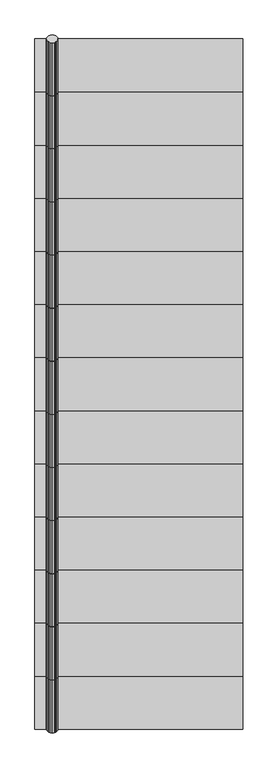
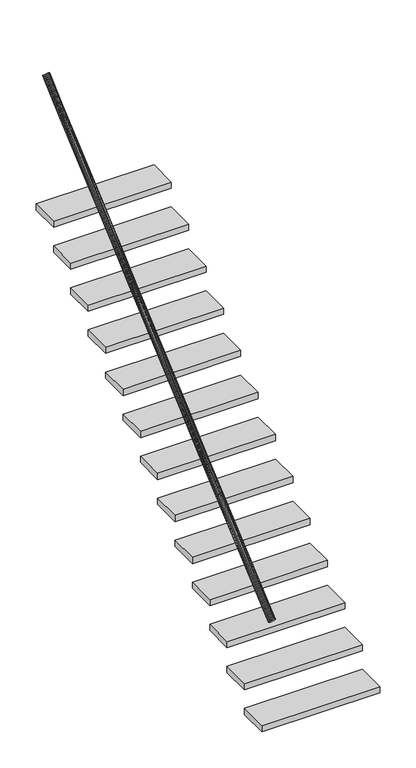
"""IFC4 building model written with IfcOpenShell, lengths in millimetres: stair geometry, 0_3d."""

from ifc_helpers import new_model, si_unit, frame, origin, origin_with_axes, place, context, project, spatial, polyline, outline, extrude, source, transform, mapped, element, save


def stair_2233e0a3(model_context):
    return source(origin(), model_context, "Body", "SweptSolid", [
        extrude(outline(polyline([(1.2235871, -7.9923214), (0.0, 0.0), (1.2235871, 7.9923214), (4.7745751, 15.2022986), (10.3053687, 20.924169), (17.2745751, 24.5978359), (25.0, 25.8636953), (32.7254249, 24.5978359), (39.6946313, 20.924169), (45.2254249, 15.2022986), (48.7764129, 7.9923214), (50.0, 0.0), (48.7764129, -7.9923214), (45.2254249, -15.2022986), (39.6946313, -20.9241691), (32.7254249, -24.5978359), (25.0, -25.8636953), (17.2745751, -24.5978359), (10.3053687, -20.9241691), (4.7745751, -15.2022986), (1.2235871, -7.9923214)])), frame((100.0, 246.9712063, 1069.5592366), z_axis=(0.0, 0.7546055221634433, 0.6561787149248571), x_axis=(-1.0, 0.0, 0.0)), (0.0, 0.0, 1.0), 304.7950131),
        extrude(outline(polyline([(1.2235871, -7.9923214), (0.0, 0.0), (1.2235871, 7.9923214), (4.7745751, 15.2022986), (10.3053687, 20.924169), (17.2745751, 24.5978359), (25.0, 25.8636953), (32.7254249, 24.5978359), (39.6946313, 20.924169), (45.2254249, 15.2022986), (48.7764129, 7.9923214), (50.0, 0.0), (48.7764129, -7.9923214), (45.2254249, -15.2022986), (39.6946313, -20.9241691), (32.7254249, -24.5978359), (25.0, -25.8636953), (17.2745751, -24.5978359), (10.3053687, -20.9241691), (4.7745751, -15.2022986), (1.2235871, -7.9923214)])), frame((100.0, 1396.9712063, 2069.5592366), z_axis=(0.0, 0.7546055221634361, 0.6561787149248655), x_axis=(-1.0, 0.0, 0.0)), (0.0, 0.0, 1.0), 304.7950131),
        extrude(outline(polyline([(0.0, 1856.9712063), (0.0, 2086.9712063), (900.0, 2086.9712063), (900.0, 1856.9712063), (0.0, 1856.9712063)])), frame((0.0, 0.0, 1600.0), z_axis=(0.0, 0.0, 1.0), x_axis=(1.0, 0.0, 0.0)), (0.0, 0.0, 1.0), 50.0),
        extrude(outline(polyline([(0.0, 2086.9712063), (0.0, 2316.9712063), (900.0, 2316.9712063), (900.0, 2086.9712063), (0.0, 2086.9712063)])), frame((0.0, 0.0, 1800.0), z_axis=(0.0, 0.0, 1.0), x_axis=(1.0, 0.0, 0.0)), (0.0, 0.0, 1.0), 50.0),
        extrude(outline(polyline([(1.2235871, -7.9923214), (0.0, 0.0), (1.2235871, 7.9923214), (4.7745751, 15.2022986), (10.3053687, 20.924169), (17.2745751, 24.5978359), (25.0, 25.8636953), (32.7254249, 24.5978359), (39.6946313, 20.924169), (45.2254249, 15.2022986), (48.7764129, 7.9923214), (50.0, 0.0), (48.7764129, -7.9923214), (45.2254249, -15.2022986), (39.6946313, -20.9241691), (32.7254249, -24.5978359), (25.0, -25.8636953), (17.2745751, -24.5978359), (10.3053687, -20.9241691), (4.7745751, -15.2022986), (1.2235871, -7.9923214)])), frame((100.0, 1166.9712063, 1869.5592366), z_axis=(0.0, 0.7546055221634385, 0.656178714924863), x_axis=(-1.0, 0.0, 0.0)), (0.0, 0.0, 1.0), 304.7950131),
        extrude(outline(polyline([(0.0, 936.9712063), (0.0, 1166.9712063), (900.0, 1166.9712063), (900.0, 936.9712063), (0.0, 936.9712063)])), frame((0.0, 0.0, 800.0), z_axis=(0.0, 0.0, 1.0), x_axis=(1.0, 0.0, 0.0)), (0.0, 0.0, 1.0), 50.0),
        extrude(outline(polyline([(0.0, 2546.9712063), (0.0, 2776.9712063), (900.0, 2776.9712063), (900.0, 2546.9712063), (0.0, 2546.9712063)])), frame((0.0, 0.0, 2200.0), z_axis=(0.0, 0.0, 1.0), x_axis=(1.0, 0.0, 0.0)), (0.0, 0.0, 1.0), 50.0),
        extrude(outline(polyline([(0.0, 1626.9712063), (0.0, 1856.9712063), (900.0, 1856.9712063), (900.0, 1626.9712063), (0.0, 1626.9712063)])), frame((0.0, 0.0, 1400.0), z_axis=(0.0, 0.0, 1.0), x_axis=(1.0, 0.0, 0.0)), (0.0, 0.0, 1.0), 50.0),
        extrude(outline(polyline([(0.0, 1166.9712063), (0.0, 1396.9712063), (900.0, 1396.9712063), (900.0, 1166.9712063), (0.0, 1166.9712063)])), frame((0.0, 0.0, 1000.0), z_axis=(0.0, 0.0, 1.0), x_axis=(1.0, 0.0, 0.0)), (0.0, 0.0, 1.0), 50.0),
        extrude(outline(polyline([(0.0, 246.9712063), (0.0, 476.9712063), (900.0, 476.9712063), (900.0, 246.9712063), (0.0, 246.9712063)])), frame((0.0, 0.0, 200.0), z_axis=(0.0, 0.0, 1.0), x_axis=(1.0, 0.0, 0.0)), (0.0, 0.0, 1.0), 50.0),
        extrude(outline(polyline([(0.0, 1396.9712063), (0.0, 1626.9712063), (900.0, 1626.9712063), (900.0, 1396.9712063), (0.0, 1396.9712063)])), frame((0.0, 0.0, 1200.0), z_axis=(0.0, 0.0, 1.0), x_axis=(1.0, 0.0, 0.0)), (0.0, 0.0, 1.0), 50.0),
        extrude(outline(polyline([(1.2235871, -7.9923214), (0.0, 0.0), (1.2235871, 7.9923214), (4.7745751, 15.2022986), (10.3053687, 20.924169), (17.2745751, 24.5978359), (25.0, 25.8636953), (32.7254249, 24.5978359), (39.6946313, 20.924169), (45.2254249, 15.2022986), (48.7764129, 7.9923214), (50.0, 0.0), (48.7764129, -7.9923214), (45.2254249, -15.2022986), (39.6946313, -20.9241691), (32.7254249, -24.5978359), (25.0, -25.8636953), (17.2745751, -24.5978359), (10.3053687, -20.9241691), (4.7745751, -15.2022986), (1.2235871, -7.9923214)])), frame((100.0, 1856.9712063, 2469.5592366), z_axis=(0.0, 0.7546055221634393, 0.6561787149248619), x_axis=(-1.0, 0.0, 0.0)), (0.0, 0.0, 1.0), 304.7950131),
        extrude(outline(polyline([(1.2235871, -7.9923214), (0.0, 0.0), (1.2235871, 7.9923214), (4.7745751, 15.2022986), (10.3053687, 20.924169), (17.2745751, 24.5978359), (25.0, 25.8636953), (32.7254249, 24.5978359), (39.6946313, 20.924169), (45.2254249, 15.2022986), (48.7764129, 7.9923214), (50.0, 0.0), (48.7764129, -7.9923214), (45.2254249, -15.2022986), (39.6946313, -20.9241691), (32.7254249, -24.5978359), (25.0, -25.8636953), (17.2745751, -24.5978359), (10.3053687, -20.9241691), (4.7745751, -15.2022986), (1.2235871, -7.9923214)])), frame((100.0, 1626.9712063, 2269.5592366), z_axis=(0.0, 0.7546055221634641, 0.6561787149248334), x_axis=(-1.0, 0.0, 0.0)), (0.0, 0.0, 1.0), 304.7950131),
        extrude(outline(polyline([(0.0, 2776.9712063), (0.0, 3006.9712063), (900.0, 3006.9712063), (900.0, 2776.9712063), (0.0, 2776.9712063)])), frame((0.0, 0.0, 2400.0), z_axis=(0.0, 0.0, 1.0), x_axis=(1.0, 0.0, 0.0)), (0.0, 0.0, 1.0), 50.0),
        extrude(outline(polyline([(0.0, 476.9712063), (0.0, 706.9712063), (900.0, 706.9712063), (900.0, 476.9712063), (0.0, 476.9712063)])), frame((0.0, 0.0, 400.0), z_axis=(0.0, 0.0, 1.0), x_axis=(1.0, 0.0, 0.0)), (0.0, 0.0, 1.0), 50.0),
        extrude(outline(polyline([(1.2235871, -7.9923214), (0.0, 0.0), (1.2235871, 7.9923214), (4.7745751, 15.2022986), (10.3053687, 20.924169), (17.2745751, 24.5978359), (25.0, 25.8636953), (32.7254249, 24.5978359), (39.6946313, 20.924169), (45.2254249, 15.2022986), (48.7764129, 7.9923214), (50.0, 0.0), (48.7764129, -7.9923214), (45.2254249, -15.2022986), (39.6946313, -20.9241691), (32.7254249, -24.5978359), (25.0, -25.8636953), (17.2745751, -24.5978359), (10.3053687, -20.9241691), (4.7745751, -15.2022986), (1.2235871, -7.9923214)])), frame((100.0, 706.9712063, 1469.5592366), z_axis=(0.0, 0.7546055221634701, 0.6561787149248264), x_axis=(-1.0, 0.0, 0.0)), (0.0, 0.0, 1.0), 304.7950131),
        extrude(outline(polyline([(1.2235871, -7.9923214), (0.0, 0.0), (1.2235871, 7.9923214), (4.7745751, 15.2022986), (10.3053687, 20.924169), (17.2745751, 24.5978359), (25.0, 25.8636953), (32.7254249, 24.5978359), (39.6946313, 20.924169), (45.2254249, 15.2022986), (48.7764129, 7.9923214), (50.0, 0.0), (48.7764129, -7.9923214), (45.2254249, -15.2022986), (39.6946313, -20.9241691), (32.7254249, -24.5978359), (25.0, -25.8636953), (17.2745751, -24.5978359), (10.3053687, -20.9241691), (4.7745751, -15.2022986), (1.2235871, -7.9923214)])), frame((100.0, 2086.9712063, 2669.5592366), z_axis=(0.0, 0.7546055221634421, 0.6561787149248586), x_axis=(-1.0, 0.0, 0.0)), (0.0, 0.0, 1.0), 304.7950131),
        extrude(outline(polyline([(1.2235871, -7.9923214), (0.0, 0.0), (1.2235871, 7.9923214), (4.7745751, 15.2022986), (10.3053687, 20.924169), (17.2745751, 24.5978359), (25.0, 25.8636953), (32.7254249, 24.5978359), (39.6946313, 20.924169), (45.2254249, 15.2022986), (48.7764129, 7.9923214), (50.0, 0.0), (48.7764129, -7.9923214), (45.2254249, -15.2022986), (39.6946313, -20.9241691), (32.7254249, -24.5978359), (25.0, -25.8636953), (17.2745751, -24.5978359), (10.3053687, -20.9241691), (4.7745751, -15.2022986), (1.2235871, -7.9923214)])), frame((100.0, 936.9712063, 1669.5592366), z_axis=(0.0, 0.7546055221634438, 0.6561787149248568), x_axis=(-1.0, 0.0, 0.0)), (0.0, 0.0, 1.0), 304.7950131),
        extrude(outline(polyline([(0.0, 706.9712063), (0.0, 936.9712063), (900.0, 936.9712063), (900.0, 706.9712063), (0.0, 706.9712063)])), frame((0.0, 0.0, 600.0), z_axis=(0.0, 0.0, 1.0), x_axis=(1.0, 0.0, 0.0)), (0.0, 0.0, 1.0), 50.0),
        extrude(outline(polyline([(1.2235871, -7.9923214), (0.0, 0.0), (1.2235871, 7.9923214), (4.7745751, 15.2022986), (10.3053687, 20.924169), (17.2745751, 24.5978359), (25.0, 25.8636953), (32.7254249, 24.5978359), (39.6946313, 20.924169), (45.2254249, 15.2022986), (48.7764129, 7.9923214), (50.0, 0.0), (48.7764129, -7.9923214), (45.2254249, -15.2022986), (39.6946313, -20.9241691), (32.7254249, -24.5978359), (25.0, -25.8636953), (17.2745751, -24.5978359), (10.3053687, -20.9241691), (4.7745751, -15.2022986), (1.2235871, -7.9923214)])), frame((100.0, 2316.9712063, 2869.5592366), z_axis=(0.0, 0.7546055221634657, 0.6561787149248317), x_axis=(-1.0, 0.0, 0.0)), (0.0, 0.0, 1.0), 304.7950131),
        extrude(outline(polyline([(1.2235871, -7.9923214), (0.0, 0.0), (1.2235871, 7.9923214), (4.7745751, 15.2022986), (10.3053687, 20.924169), (17.2745751, 24.5978359), (25.0, 25.8636953), (32.7254249, 24.5978359), (39.6946313, 20.924169), (45.2254249, 15.2022986), (48.7764129, 7.9923214), (50.0, 0.0), (48.7764129, -7.9923214), (45.2254249, -15.2022986), (39.6946313, -20.9241691), (32.7254249, -24.5978359), (25.0, -25.8636953), (17.2745751, -24.5978359), (10.3053687, -20.9241691), (4.7745751, -15.2022986), (1.2235871, -7.9923214)])), frame((100.0, 2776.9712063, 3269.5592366), z_axis=(0.0, 0.754605522163467, 0.65617871492483), x_axis=(-1.0, 0.0, 0.0)), (0.0, 0.0, 1.0), 304.7950131),
        extrude(outline(polyline([(1.2235871, -7.9923214), (0.0, 0.0), (1.2235871, 7.9923214), (4.7745751, 15.2022986), (10.3053687, 20.924169), (17.2745751, 24.5978359), (25.0, 25.8636953), (32.7254249, 24.5978359), (39.6946313, 20.924169), (45.2254249, 15.2022986), (48.7764129, 7.9923214), (50.0, 0.0), (48.7764129, -7.9923214), (45.2254249, -15.2022986), (39.6946313, -20.9241691), (32.7254249, -24.5978359), (25.0, -25.8636953), (17.2745751, -24.5978359), (10.3053687, -20.9241691), (4.7745751, -15.2022986), (1.2235871, -7.9923214)])), frame((100.0, 476.9712063, 1269.5592366), z_axis=(0.0, 0.7546055221634442, 0.6561787149248562), x_axis=(-1.0, 0.0, 0.0)), (0.0, 0.0, 1.0), 304.7950131),
        extrude(outline(polyline([(0.0, 2316.9712063), (0.0, 2546.9712063), (900.0, 2546.9712063), (900.0, 2316.9712063), (0.0, 2316.9712063)])), frame((0.0, 0.0, 2000.0), z_axis=(0.0, 0.0, 1.0), x_axis=(1.0, 0.0, 0.0)), (0.0, 0.0, 1.0), 50.0),
        extrude(outline(polyline([(0.0, 16.9712063), (0.0, 246.9712063), (900.0, 246.9712063), (900.0, 16.9712063), (0.0, 16.9712063)])), origin_with_axes(), (0.0, 0.0, 1.0), 50.0),
        extrude(outline(polyline([(1.2235871, -7.9923214), (0.0, 0.0), (1.2235871, 7.9923214), (4.7745751, 15.2022986), (10.3053687, 20.924169), (17.2745751, 24.5978359), (25.0, 25.8636953), (32.7254249, 24.5978359), (39.6946313, 20.924169), (45.2254249, 15.2022986), (48.7764129, 7.9923214), (50.0, 0.0), (48.7764129, -7.9923214), (45.2254249, -15.2022986), (39.6946313, -20.9241691), (32.7254249, -24.5978359), (25.0, -25.8636953), (17.2745751, -24.5978359), (10.3053687, -20.9241691), (4.7745751, -15.2022986), (1.2235871, -7.9923214)])), frame((100.0, 2546.9712063, 3069.5592366), z_axis=(0.0, 0.7546055221634356, 0.6561787149248662), x_axis=(-1.0, 0.0, 0.0)), (0.0, 0.0, 1.0), 304.7950131),
        extrude(outline(polyline([(1.2235871, -7.9923214), (0.0, 0.0), (1.2235871, 7.9923214), (4.7745751, 15.2022986), (10.3053687, 20.924169), (17.2745751, 24.5978359), (25.0, 25.8636953), (32.7254249, 24.5978359), (39.6946313, 20.924169), (45.2254249, 15.2022986), (48.7764129, 7.9923214), (50.0, 0.0), (48.7764129, -7.9923214), (45.2254249, -15.2022986), (39.6946313, -20.9241691), (32.7254249, -24.5978359), (25.0, -25.8636953), (17.2745751, -24.5978359), (10.3053687, -20.9241691), (4.7745751, -15.2022986), (1.2235871, -7.9923214)])), frame((100.0, 16.9712063, 869.5592366), z_axis=(0.0, 0.7546055221634935, 0.6561787149247995), x_axis=(-1.0, 0.0, 0.0)), (0.0, 0.0, 1.0), 304.7950131),
    ])


if __name__ == "__main__":
    model = new_model("IFC4")
    model_context = context("Model", 3, world=origin())
    ifc_project = project(units=[si_unit("LENGTHUNIT", "METRE", prefix="MILLI")], contexts=[model_context])
    site = spatial("IfcSite", under=ifc_project)
    building = spatial("IfcBuilding", under=site)
    placement = place(None, origin())
    stair_shape = stair_2233e0a3(model_context)
    element("IfcStair", 1, ObjectType="0_3d", at=placement, inside=building, context=model_context, shape_type="MappedRepresentation", body=[
        mapped(stair_shape, transform((0.0, 0.0, 0.0), x_axis=(1.0, 0.0, 0.0), y_axis=(0.0, 1.0, 0.0), z_axis=(0.0, 0.0, 1.0))),
    ])
    save(model, "model.ifc")

# Revit data of these elements
# Element 1 (IfcStair, "0_3d")
#   Materials on its faces: "*1", "weiss"
# Materials
#   "*1": class "Unassigned", colour RGB 175 175 175, transparency 0
#   "weiss": class "Unassigned", colour RGB 255 255 255, transparency 0
